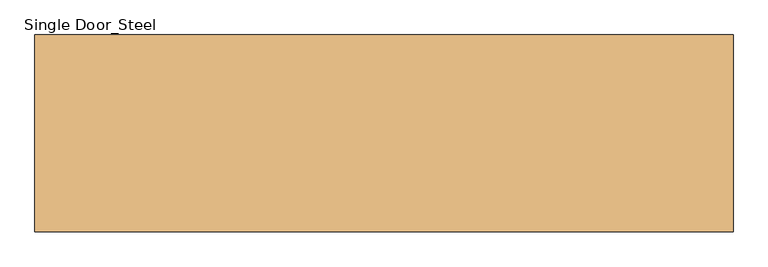
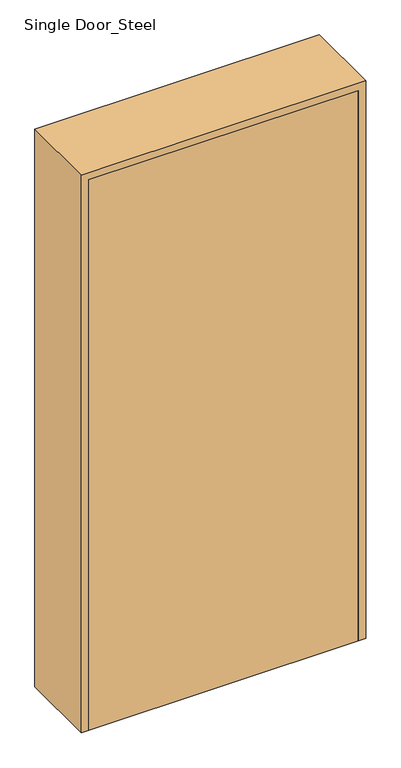
"""IFC4 building model written with IfcOpenShell, lengths in millimetres: door geometry, Single Door_Steel : H_DR_AR_B12_Single Door_Steel_W1100xH2280_SD1."""

import ifcopenshell
import ifcopenshell.guid

model = None  # the IFC model being written
_history = None  # IfcOwnerHistory: only IFC2X3 demands one
_inside = {}  # id of a spatial element -> (the spatial element, [elements in it])
_under = {}  # id of a project, library or spatial element -> (it, [spatial elements below it])
_declared = {}  # id of a project -> (the project, [libraries it declares])
_typed = {}  # id of a type object -> (the type object, [elements of that type])
_made_of = {}  # id of a material, layer set ... -> (it, [elements and type objects made of it])


def new_model(schema):
    """Start an empty IFC model of exactly this schema.

    Asked for "IFC4X3", IfcOpenShell would pick the latest addendum, in which some entities
    have other attributes; the version numbers below select the first issue.
    IFC2X3 requires an IfcOwnerHistory on every rooted entity: one is made here for all.
    """
    global model, _history
    if schema == "IFC4X3":
        model = ifcopenshell.file(schema_version=(4, 3, 0, 0))
    else:
        model = ifcopenshell.file(schema=schema)
    _inside.clear()
    _under.clear()
    _declared.clear()
    _typed.clear()
    _made_of.clear()
    _history = None
    if model.schema == "IFC2X3":
        org = make("IfcOrganization", Name="unknown")
        user = make(
            "IfcPersonAndOrganization",
            ThePerson=make("IfcPerson", FamilyName="unknown"),
            TheOrganization=org,
        )
        app = make(
            "IfcApplication",
            ApplicationDeveloper=org,
            Version="unknown",
            ApplicationFullName="unknown",
            ApplicationIdentifier="unknown",
        )
        _history = make(
            "IfcOwnerHistory",
            OwningUser=user,
            OwningApplication=app,
            ChangeAction="ADDED",
            CreationDate=0,
        )
    return model


def make(cls, **values):
    """One entity of the class cls with the attributes given. An attribute that is None is left unset."""
    return model.create_entity(
        cls, **{name: value for name, value in values.items() if value is not None}
    )


def rooted(cls, **values):
    """An entity with a GlobalId (a new one), such as an element, a storey or a relation."""
    return make(cls, GlobalId=ifcopenshell.guid.new(), OwnerHistory=_history, **values)


def si_unit(unit_type, name, prefix=None):
    """IfcSIUnit, for example si_unit("LENGTHUNIT", "METRE", prefix="MILLI")."""
    return make("IfcSIUnit", UnitType=unit_type, Prefix=prefix, Name=name)


def assignment(units):
    """IfcUnitAssignment: the units of a project."""
    return None if units is None else make("IfcUnitAssignment", Units=units)


def point(xyz):
    """IfcCartesianPoint."""
    return None if xyz is None else make("IfcCartesianPoint", Coordinates=xyz)


def direction(xyz):
    """IfcDirection."""
    return None if xyz is None else make("IfcDirection", DirectionRatios=xyz)


def frame(location, z_axis=None, x_axis=None):
    """IfcAxis2Placement3D, a coordinate frame: its origin and axes. An axis left out is left unset."""
    return make(
        "IfcAxis2Placement3D",
        Location=point(location),
        Axis=direction(z_axis),
        RefDirection=direction(x_axis),
    )


def origin():
    """The frame at (0, 0, 0) with its axes left unset."""
    return frame((0.0, 0.0, 0.0))


def origin_with_axes():
    """The frame at (0, 0, 0) with the z axis (0, 0, 1) and the x axis (1, 0, 0) written out."""
    return frame((0.0, 0.0, 0.0), z_axis=(0.0, 0.0, 1.0), x_axis=(1.0, 0.0, 0.0))


def place(relative_to, where):
    """IfcLocalPlacement: puts the frame where relative to a parent placement (None: the world)."""
    return make(
        "IfcLocalPlacement", PlacementRelTo=relative_to, RelativePlacement=where
    )


def context(
    kind, dimensions, precision=None, world=None, true_north=None, identifier=None
):
    """IfcGeometricRepresentationContext, for example the 3D "Model" context."""
    return make(
        "IfcGeometricRepresentationContext",
        ContextIdentifier=identifier,
        ContextType=kind,
        CoordinateSpaceDimension=dimensions,
        Precision=precision,
        WorldCoordinateSystem=world,
        TrueNorth=true_north,
    )


def project(units=None, contexts=None):
    """IfcProject with its units and contexts."""
    return rooted(
        "IfcProject",
        Name="project",
        RepresentationContexts=contexts,
        UnitsInContext=assignment(units),
    )


def spatial(cls, under=None, at=None, **own):
    """A site, building, storey or space (cls), placed at a placement, below another one or the project."""
    s = rooted(cls, ObjectPlacement=at, **own)
    if under is not None:
        _under.setdefault(under.id(), (under, []))[1].append(s)
    return s


def polyline(points):
    """IfcPolyline through the points."""
    return make("IfcPolyline", Points=[point(p) for p in points])


def outline(outer, holes=None, kind="AREA"):
    """IfcArbitraryClosedProfileDef: a profile drawn as a closed curve; with holes, ...WithVoids."""
    if holes is None:
        return make("IfcArbitraryClosedProfileDef", ProfileType=kind, OuterCurve=outer)
    return make(
        "IfcArbitraryProfileDefWithVoids",
        ProfileType=kind,
        OuterCurve=outer,
        InnerCurves=holes,
    )


def extrude(swept, where, along, depth):
    """IfcExtrudedAreaSolid: the profile swept, set in the frame where, extruded along a direction by depth."""
    return make(
        "IfcExtrudedAreaSolid",
        SweptArea=swept,
        Position=where,
        ExtrudedDirection=direction(along),
        Depth=depth,
    )


def faces_of(points, faces, orient=None, outer=None):
    """IfcFace entities. A face is a list of loops; a loop is a list of indices into points, from 0.

    orient and outer hold one flag for each loop. By default every Orientation is true, the
    first loop of a face is its IfcFaceOuterBound and the others are IfcFaceBound.
    """
    made = []
    for i, loops in enumerate(faces):
        bounds = []
        for j, loop in enumerate(loops):
            is_outer = j == 0 if outer is None else outer[i][j]
            bounds.append(
                make(
                    "IfcFaceOuterBound" if is_outer else "IfcFaceBound",
                    Bound=make("IfcPolyLoop", Polygon=[points[k] for k in loop]),
                    Orientation=True if orient is None else orient[i][j],
                )
            )
        made.append(make("IfcFace", Bounds=bounds))
    return made


def faceted_brep(points, faces, orient=None, outer=None, voids=None):
    """IfcFacetedBrep: a solid bounded by flat faces; with voids (closed shells), ...WithVoids."""
    shared = [point(p) for p in points]
    hull = make("IfcClosedShell", CfsFaces=faces_of(shared, faces, orient, outer))
    if voids is None:
        return make("IfcFacetedBrep", Outer=hull)
    return make(
        "IfcFacetedBrepWithVoids",
        Outer=hull,
        Voids=[
            make(cls, CfsFaces=faces_of(shared, fs, o, b)) for cls, fs, o, b in voids
        ],
    )


def shape(context_of_items, identifier, shape_type, items):
    """IfcShapeRepresentation: the items that make up one representation, for example the "Body"."""
    return make(
        "IfcShapeRepresentation",
        ContextOfItems=context_of_items,
        RepresentationIdentifier=identifier,
        RepresentationType=shape_type,
        Items=items,
    )


def source(mapping_origin, context_of_items, identifier, shape_type, items):
    """IfcRepresentationMap: a shape defined once, which mapped items show again and again."""
    return make(
        "IfcRepresentationMap",
        MappingOrigin=mapping_origin,
        MappedRepresentation=shape(context_of_items, identifier, shape_type, items),
    )


def transform(
    local_origin,
    x_axis=None,
    y_axis=None,
    z_axis=None,
    scale=None,
    scale2=None,
    scale3=None,
    uniform=True,
):
    """IfcCartesianTransformationOperator3D, or its non-uniform kind. x_axis, y_axis, z_axis: its Axis1, 2, 3."""
    if uniform:
        return make(
            "IfcCartesianTransformationOperator3D",
            Axis1=direction(x_axis),
            Axis2=direction(y_axis),
            LocalOrigin=point(local_origin),
            Scale=scale,
            Axis3=direction(z_axis),
        )
    return make(
        "IfcCartesianTransformationOperator3DnonUniform",
        Axis1=direction(x_axis),
        Axis2=direction(y_axis),
        LocalOrigin=point(local_origin),
        Scale=scale,
        Axis3=direction(z_axis),
        Scale2=scale2,
        Scale3=scale3,
    )


def mapped(mapping_source, mapping_target):
    """IfcMappedItem: shows the shape of a source again, moved by a transform."""
    return make(
        "IfcMappedItem", MappingSource=mapping_source, MappingTarget=mapping_target
    )


def made_of(thing, what):
    """Note that an element or type object is made of a material, layer set ...; save() writes the relation."""
    if what is not None:
        _made_of.setdefault(what.id(), (what, []))[1].append(thing)
    return thing


def element(
    cls,
    number,
    at=None,
    inside=None,
    cuts=None,
    type_object=None,
    material=None,
    context=None,
    identifier="Body",
    shape_type=None,
    held_by="IfcProductDefinitionShape",
    body=None,
    shapes=None,
    **own,
):
    """One element of the class cls, such as IfcWall. Its Tag is "e" and its number.

    at: its placement. inside: the storey or other place that contains it. cuts: it is an
    opening in that element (IfcRelVoidsElement). A single representation is given by context,
    identifier, shape_type and body (its items); several are given by shapes. held_by: the class
    of the entity that holds the representations. save() writes the other relations.
    """
    e = rooted(cls, Tag="e%d" % number, ObjectPlacement=at, **own)
    if body is not None:
        shapes = [shape(context, identifier, shape_type, body)]
    if shapes is not None:
        e.Representation = make(held_by, Representations=shapes)
    if inside is not None:
        _inside.setdefault(inside.id(), (inside, []))[1].append(e)
    if cuts is not None:
        rooted(
            "IfcRelVoidsElement", RelatingBuildingElement=cuts, RelatedOpeningElement=e
        )
    if type_object is not None:
        _typed.setdefault(type_object.id(), (type_object, []))[1].append(e)
    return made_of(e, material)


def aggregate(whole, parts):
    """IfcRelAggregates: a whole, such as a stair, and the parts it consists of."""
    return rooted("IfcRelAggregates", RelatingObject=whole, RelatedObjects=parts)


def save(model, path):
    """Write the relations noted so far, then the file.

    IfcRelAggregates (storeys below a building ...), IfcRelContainedInSpatialStructure (elements
    in a storey), IfcRelDefinesByType, IfcRelAssociatesMaterial and IfcRelDeclares: one each for
    every whole, place, type object, material and project.
    """
    for whole, parts in _under.values():
        aggregate(whole, parts)
    for where, things in _inside.values():
        rooted(
            "IfcRelContainedInSpatialStructure",
            RelatedElements=things,
            RelatingStructure=where,
        )
    for kind, things in _typed.values():
        rooted("IfcRelDefinesByType", RelatedObjects=things, RelatingType=kind)
    for what, things in _made_of.values():
        rooted("IfcRelAssociatesMaterial", RelatedObjects=things, RelatingMaterial=what)
    for by, libraries in _declared.values():
        rooted("IfcRelDeclares", RelatingContext=by, RelatedDefinitions=libraries)
    model.write(path)


def single_door_steel_0719061a(model_context):
    return source(origin(), model_context, "Body", "SolidModel", [
        extrude(outline(polyline([(520.0, -155.0), (-520.0, -155.0), (-520.0, -120.0), (520.0, -120.0), (520.0, -155.0)])), origin_with_axes(), (0.0, 0.0, 1.0), 2250.0),
        faceted_brep([(520.0, -155.0, 0.0), (520.0, -120.0, 0.0), (500.0, -120.0, 0.0), (500.0, 120.0, 0.0), (520.0, 120.0, 0.0), (520.0, 155.0, 0.0), (550.0, 155.0, 0.0), (550.0, -155.0, 0.0), (550.0, -155.0, 2280.0), (-550.0, -155.0, 2280.0), (-550.0, -155.0, 0.0), (-520.0, -155.0, 0.0), (-520.0, -155.0, 2250.0), (520.0, -155.0, 2250.0), (550.0, 155.0, 2280.0), (520.0, 155.0, 2250.0), (-520.0, 155.0, 2250.0), (-520.0, 155.0, 0.0), (-550.0, 155.0, 0.0), (-550.0, 155.0, 2280.0), (520.0, 120.0, 2250.0), (500.0, 120.0, 2230.0), (-500.0, 120.0, 2230.0), (-500.0, 120.0, 0.0), (-520.0, 120.0, 0.0), (-520.0, 120.0, 2250.0), (500.0, -120.0, 2230.0), (520.0, -120.0, 2250.0), (-520.0, -120.0, 2250.0), (-520.0, -120.0, 0.0), (-500.0, -120.0, 0.0), (-500.0, -120.0, 2230.0)], [[[0, 1, 2, 3, 4, 5, 6, 7]], [[7, 8, 9, 10, 11, 12, 13, 0]], [[6, 14, 8, 7]], [[5, 15, 16, 17, 18, 19, 14, 6]], [[4, 20, 15, 5]], [[3, 21, 22, 23, 24, 25, 20, 4]], [[2, 26, 21, 3]], [[1, 27, 28, 29, 30, 31, 26, 2]], [[0, 13, 27, 1]], [[12, 11, 29, 28]], [[11, 10, 18, 17, 24, 23, 30, 29]], [[19, 18, 10, 9]], [[25, 24, 17, 16]], [[31, 30, 23, 22]], [[14, 19, 9, 8]], [[20, 25, 16, 15]], [[26, 31, 22, 21]], [[13, 12, 28, 27]]]),
    ])


if __name__ == "__main__":
    model = new_model("IFC4")
    model_context = context("Model", 3, world=origin())
    ifc_project = project(units=[si_unit("LENGTHUNIT", "METRE", prefix="MILLI")], contexts=[model_context])
    site = spatial("IfcSite", under=ifc_project)
    building = spatial("IfcBuilding", under=site)
    placement = place(None, origin())
    single_door_steel_shape = single_door_steel_0719061a(model_context)
    element("IfcDoor", 1, ObjectType="Single Door_Steel : H_DR_AR_B12_Single Door_Steel_W1100xH2280_SD1", at=placement, inside=building, context=model_context, shape_type="MappedRepresentation", body=[
        mapped(single_door_steel_shape, transform((0.0, 0.0, 0.0), x_axis=(1.0, 0.0, 0.0), y_axis=(0.0, 1.0, 0.0), z_axis=(0.0, 0.0, 1.0))),
    ])
    save(model, "model.ifc")

# Revit data of these elements
# Type "Single Door_Steel : H_DR_AR_B12_Single Door_Steel_W1100xH2280_SD1"
#   Type Mark = "430"
#   Analytic Construction = "<None>"
#   프레임 투영 외부. = 25 mm
#   프레임 투영 내부. = 25 mm
#   프레임 폭 = 75 mm
#   Height = 2280 mm
#   Width = 1100 mm
#   Define Thermal Properties by = 1
#   문 패널 = none
#   문 프레임 = none
#   Function = (empty or 0)
#   Wall Closure = (empty or 0)
